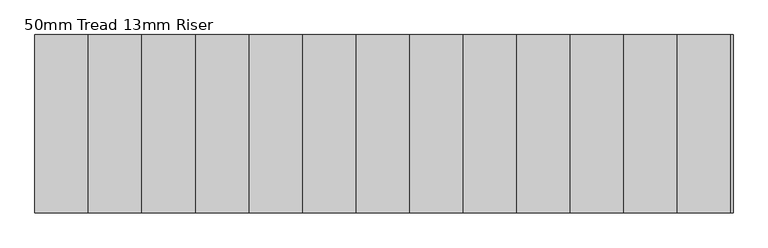
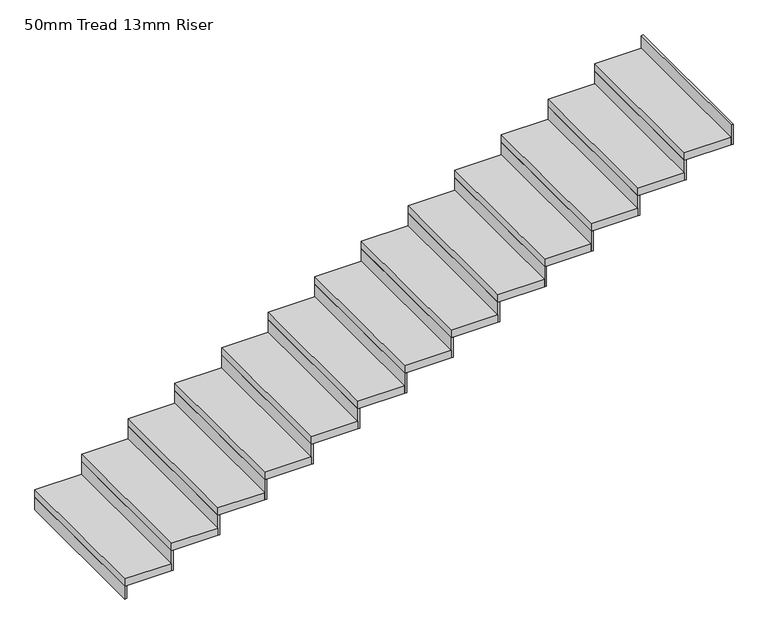
"""IFC4 building model written with IfcOpenShell, lengths in millimetres: stair flight geometry, 50mm Tread 13mm Riser."""

from ifc_helpers import new_model, si_unit, frame, origin, origin_with_axes, place, context, project, spatial, polyline, outline, extrude, source, transform, mapped, element, save


def stair_flight_50mm_tread_13mm_riser_28c962cd(model_context):
    return source(origin(), model_context, "Body", "SweptSolid", [
        extrude(outline(polyline([(17662.336337, -4576.2808257), (17649.836337, -4576.2808257), (17649.836337, -3576.2808257), (17662.336337, -3576.2808257), (17662.336337, -4576.2808257)])), origin_with_axes(), (0.0, 0.0, 1.0), 86.3636364),
        extrude(outline(polyline([(17949.836337, -3576.2808257), (17949.836337, -4576.2808257), (17649.836337, -4576.2808257), (17649.836337, -3576.2808257), (17949.836337, -3576.2808257)])), frame((0.0, 0.0, 86.3636364), z_axis=(0.0, 0.0, 1.0), x_axis=(1.0, 0.0, 0.0)), (0.0, 0.0, 1.0), 50.0),
        extrude(outline(polyline([(17962.336337, -4576.2808257), (17949.836337, -4576.2808257), (17949.836337, -3576.2808257), (17962.336337, -3576.2808257), (17962.336337, -4576.2808257)])), frame((0.0, 0.0, 86.3636364), z_axis=(0.0, 0.0, 1.0), x_axis=(1.0, 0.0, 0.0)), (0.0, 0.0, 1.0), 136.3636364),
        extrude(outline(polyline([(18249.836337, -3576.2808257), (18249.836337, -4576.2808257), (17949.836337, -4576.2808257), (17949.836337, -3576.2808257), (18249.836337, -3576.2808257)])), frame((0.0, 0.0, 222.7272727), z_axis=(0.0, 0.0, 1.0), x_axis=(1.0, 0.0, 0.0)), (0.0, 0.0, 1.0), 50.0),
        extrude(outline(polyline([(18262.336337, -4576.2808257), (18249.836337, -4576.2808257), (18249.836337, -3576.2808257), (18262.336337, -3576.2808257), (18262.336337, -4576.2808257)])), frame((0.0, 0.0, 222.7272727), z_axis=(0.0, 0.0, 1.0), x_axis=(1.0, 0.0, 0.0)), (0.0, 0.0, 1.0), 136.3636364),
        extrude(outline(polyline([(18549.836337, -3576.2808257), (18549.836337, -4576.2808257), (18249.836337, -4576.2808257), (18249.836337, -3576.2808257), (18549.836337, -3576.2808257)])), frame((0.0, 0.0, 359.0909091), z_axis=(0.0, 0.0, 1.0), x_axis=(1.0, 0.0, 0.0)), (0.0, 0.0, 1.0), 50.0),
        extrude(outline(polyline([(18562.336337, -4576.2808257), (18549.836337, -4576.2808257), (18549.836337, -3576.2808257), (18562.336337, -3576.2808257), (18562.336337, -4576.2808257)])), frame((0.0, 0.0, 359.0909091), z_axis=(0.0, 0.0, 1.0), x_axis=(1.0, 0.0, 0.0)), (0.0, 0.0, 1.0), 136.3636364),
        extrude(outline(polyline([(18849.836337, -3576.2808257), (18849.836337, -4576.2808257), (18549.836337, -4576.2808257), (18549.836337, -3576.2808257), (18849.836337, -3576.2808257)])), frame((0.0, 0.0, 495.4545455), z_axis=(0.0, 0.0, 1.0), x_axis=(1.0, 0.0, 0.0)), (0.0, 0.0, 1.0), 50.0),
        extrude(outline(polyline([(18862.336337, -4576.2808257), (18849.836337, -4576.2808257), (18849.836337, -3576.2808257), (18862.336337, -3576.2808257), (18862.336337, -4576.2808257)])), frame((0.0, 0.0, 495.4545455), z_axis=(0.0, 0.0, 1.0), x_axis=(1.0, 0.0, 0.0)), (0.0, 0.0, 1.0), 136.3636364),
        extrude(outline(polyline([(19149.836337, -3576.2808257), (19149.836337, -4576.2808257), (18849.836337, -4576.2808257), (18849.836337, -3576.2808257), (19149.836337, -3576.2808257)])), frame((0.0, 0.0, 631.8181818), z_axis=(0.0, 0.0, 1.0), x_axis=(1.0, 0.0, 0.0)), (0.0, 0.0, 1.0), 50.0),
        extrude(outline(polyline([(19162.336337, -4576.2808257), (19149.836337, -4576.2808257), (19149.836337, -3576.2808257), (19162.336337, -3576.2808257), (19162.336337, -4576.2808257)])), frame((0.0, 0.0, 631.8181818), z_axis=(0.0, 0.0, 1.0), x_axis=(1.0, 0.0, 0.0)), (0.0, 0.0, 1.0), 136.3636364),
        extrude(outline(polyline([(19449.836337, -3576.2808257), (19449.836337, -4576.2808257), (19149.836337, -4576.2808257), (19149.836337, -3576.2808257), (19449.836337, -3576.2808257)])), frame((0.0, 0.0, 768.1818182), z_axis=(0.0, 0.0, 1.0), x_axis=(1.0, 0.0, 0.0)), (0.0, 0.0, 1.0), 50.0),
        extrude(outline(polyline([(19462.336337, -4576.2808257), (19449.836337, -4576.2808257), (19449.836337, -3576.2808257), (19462.336337, -3576.2808257), (19462.336337, -4576.2808257)])), frame((0.0, 0.0, 768.1818182), z_axis=(0.0, 0.0, 1.0), x_axis=(1.0, 0.0, 0.0)), (0.0, 0.0, 1.0), 136.3636364),
        extrude(outline(polyline([(19749.836337, -3576.2808257), (19749.836337, -4576.2808257), (19449.836337, -4576.2808257), (19449.836337, -3576.2808257), (19749.836337, -3576.2808257)])), frame((0.0, 0.0, 904.5454545), z_axis=(0.0, 0.0, 1.0), x_axis=(1.0, 0.0, 0.0)), (0.0, 0.0, 1.0), 50.0),
        extrude(outline(polyline([(19762.336337, -4576.2808257), (19749.836337, -4576.2808257), (19749.836337, -3576.2808257), (19762.336337, -3576.2808257), (19762.336337, -4576.2808257)])), frame((0.0, 0.0, 904.5454545), z_axis=(0.0, 0.0, 1.0), x_axis=(1.0, 0.0, 0.0)), (0.0, 0.0, 1.0), 136.3636364),
        extrude(outline(polyline([(20049.836337, -3576.2808257), (20049.836337, -4576.2808257), (19749.836337, -4576.2808257), (19749.836337, -3576.2808257), (20049.836337, -3576.2808257)])), frame((0.0, 0.0, 1040.9090909), z_axis=(0.0, 0.0, 1.0), x_axis=(1.0, 0.0, 0.0)), (0.0, 0.0, 1.0), 50.0),
        extrude(outline(polyline([(20062.336337, -4576.2808257), (20049.836337, -4576.2808257), (20049.836337, -3576.2808257), (20062.336337, -3576.2808257), (20062.336337, -4576.2808257)])), frame((0.0, 0.0, 1040.9090909), z_axis=(0.0, 0.0, 1.0), x_axis=(1.0, 0.0, 0.0)), (0.0, 0.0, 1.0), 136.3636364),
        extrude(outline(polyline([(20349.836337, -3576.2808257), (20349.836337, -4576.2808257), (20049.836337, -4576.2808257), (20049.836337, -3576.2808257), (20349.836337, -3576.2808257)])), frame((0.0, 0.0, 1177.2727273), z_axis=(0.0, 0.0, 1.0), x_axis=(1.0, 0.0, 0.0)), (0.0, 0.0, 1.0), 50.0),
        extrude(outline(polyline([(20362.336337, -4576.2808257), (20349.836337, -4576.2808257), (20349.836337, -3576.2808257), (20362.336337, -3576.2808257), (20362.336337, -4576.2808257)])), frame((0.0, 0.0, 1177.2727273), z_axis=(0.0, 0.0, 1.0), x_axis=(1.0, 0.0, 0.0)), (0.0, 0.0, 1.0), 136.3636364),
        extrude(outline(polyline([(20649.836337, -3576.2808257), (20649.836337, -4576.2808257), (20349.836337, -4576.2808257), (20349.836337, -3576.2808257), (20649.836337, -3576.2808257)])), frame((0.0, 0.0, 1313.6363636), z_axis=(0.0, 0.0, 1.0), x_axis=(1.0, 0.0, 0.0)), (0.0, 0.0, 1.0), 50.0),
        extrude(outline(polyline([(20662.336337, -4576.2808257), (20649.836337, -4576.2808257), (20649.836337, -3576.2808257), (20662.336337, -3576.2808257), (20662.336337, -4576.2808257)])), frame((0.0, 0.0, 1313.6363636), z_axis=(0.0, 0.0, 1.0), x_axis=(1.0, 0.0, 0.0)), (0.0, 0.0, 1.0), 136.3636364),
        extrude(outline(polyline([(20949.836337, -3576.2808257), (20949.836337, -4576.2808257), (20649.836337, -4576.2808257), (20649.836337, -3576.2808257), (20949.836337, -3576.2808257)])), frame((0.0, 0.0, 1450.0), z_axis=(0.0, 0.0, 1.0), x_axis=(1.0, 0.0, 0.0)), (0.0, 0.0, 1.0), 50.0),
        extrude(outline(polyline([(20962.336337, -4576.2808257), (20949.836337, -4576.2808257), (20949.836337, -3576.2808257), (20962.336337, -3576.2808257), (20962.336337, -4576.2808257)])), frame((0.0, 0.0, 1450.0), z_axis=(0.0, 0.0, 1.0), x_axis=(1.0, 0.0, 0.0)), (0.0, 0.0, 1.0), 136.3636364),
        extrude(outline(polyline([(21249.836337, -3576.2808257), (21249.836337, -4576.2808257), (20949.836337, -4576.2808257), (20949.836337, -3576.2808257), (21249.836337, -3576.2808257)])), frame((0.0, 0.0, 1586.3636364), z_axis=(0.0, 0.0, 1.0), x_axis=(1.0, 0.0, 0.0)), (0.0, 0.0, 1.0), 50.0),
        extrude(outline(polyline([(21262.336337, -4576.2808257), (21249.836337, -4576.2808257), (21249.836337, -3576.2808257), (21262.336337, -3576.2808257), (21262.336337, -4576.2808257)])), frame((0.0, 0.0, 1586.3636364), z_axis=(0.0, 0.0, 1.0), x_axis=(1.0, 0.0, 0.0)), (0.0, 0.0, 1.0), 136.3636364),
        extrude(outline(polyline([(21562.336337, -4576.2808257), (21549.836337, -4576.2808257), (21549.836337, -3576.2808257), (21562.336337, -3576.2808257), (21562.336337, -4576.2808257)])), frame((0.0, 0.0, 1722.7272727), z_axis=(0.0, 0.0, 1.0), x_axis=(1.0, 0.0, 0.0)), (0.0, 0.0, 1.0), 136.3636364),
        extrude(outline(polyline([(21549.836337, -3576.2808257), (21549.836337, -4576.2808257), (21249.836337, -4576.2808257), (21249.836337, -3576.2808257), (21549.836337, -3576.2808257)])), frame((0.0, 0.0, 1722.7272727), z_axis=(0.0, 0.0, 1.0), x_axis=(1.0, 0.0, 0.0)), (0.0, 0.0, 1.0), 50.0),
    ])


if __name__ == "__main__":
    model = new_model("IFC4")
    model_context = context("Model", 3, world=origin())
    ifc_project = project(units=[si_unit("LENGTHUNIT", "METRE", prefix="MILLI")], contexts=[model_context])
    site = spatial("IfcSite", under=ifc_project)
    building = spatial("IfcBuilding", under=site)
    placement = place(None, origin())
    stair_flight_50mm_tread_13mm_riser_shape = stair_flight_50mm_tread_13mm_riser_28c962cd(model_context)
    element("IfcStairFlight", 1, ObjectType="50mm Tread 13mm Riser", at=placement, inside=building, context=model_context, shape_type="MappedRepresentation", body=[
        mapped(stair_flight_50mm_tread_13mm_riser_shape, transform((0.0, 0.0, 0.0), x_axis=(1.0, 0.0, 0.0), y_axis=(0.0, 1.0, 0.0), z_axis=(0.0, 0.0, 1.0))),
    ])
    save(model, "model.ifc")
